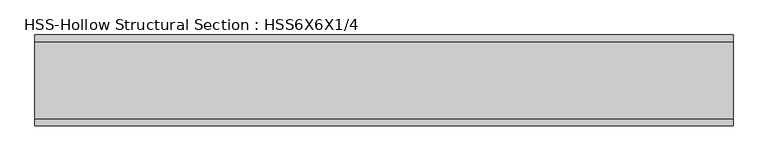
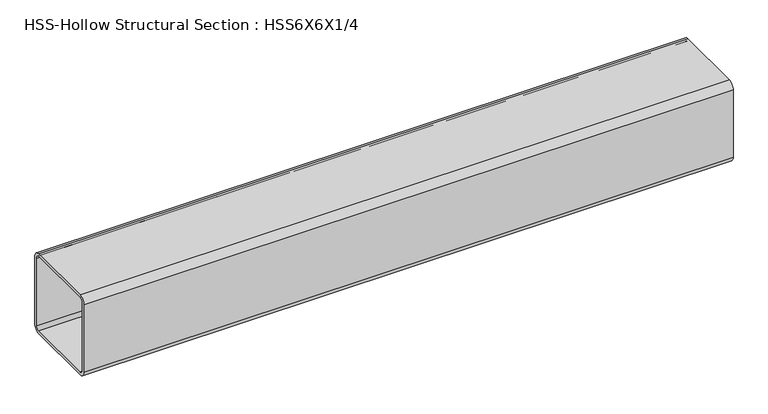
"""IFC4 building model written with IfcOpenShell, lengths in millimetres: beam geometry, HSS-Hollow Structural Section : HSS6X6X1/4."""

from ifc_helpers import new_model, si_unit, point, frame, frame_2d, origin, place, context, project, spatial, polyline, circle_curve, trimmed, segment, composite_curve, outline, extrude, source, transform, mapped, element, save


def hss_hollow_structural_section_hss6x6x1_4_3c38727f(model_context):
    return source(origin(), model_context, "Body", "SweptSolid", [
        extrude(outline(composite_curve([segment(polyline([(76.2, 64.3636), (76.2, -64.3636)]), True, "CONTINUOUS"), segment(trimmed(circle_curve(frame_2d((64.3636, -64.3636)), 11.8364), [point((76.2, -64.3636))], [point((64.3636, -76.2))], False, "CARTESIAN"), True, "CONTINUOUS"), segment(polyline([(64.3636, -76.2), (-64.3636, -76.2)]), True, "CONTINUOUS"), segment(trimmed(circle_curve(frame_2d((-64.3636, -64.3636)), 11.8364), [point((-64.3636, -76.2))], [point((-76.2, -64.3636))], False, "CARTESIAN"), True, "CONTINUOUS"), segment(polyline([(-76.2, -64.3636), (-76.2, 64.3636)]), True, "CONTINUOUS"), segment(trimmed(circle_curve(frame_2d((-64.3636, 64.3636)), 11.8364), [point((-76.2, 64.3636))], [point((-64.3636, 76.2))], False, "CARTESIAN"), True, "CONTINUOUS"), segment(polyline([(-64.3636, 76.2), (64.3636, 76.2)]), True, "CONTINUOUS"), segment(trimmed(circle_curve(frame_2d((64.3636, 64.3636)), 11.8364), [point((64.3636, 76.2))], [point((76.2, 64.3636))], False, "CARTESIAN"), True, "CONTINUOUS")], self_intersect=False), holes=[composite_curve([segment(trimmed(circle_curve(frame_2d((-64.3636, 64.3636)), 5.9182), [point((-64.3636, 70.2818))], [point((-70.2818, 64.3636))], True, "CARTESIAN"), True, "CONTINUOUS"), segment(polyline([(-70.2818, 64.3636), (-70.2818, -64.3636)]), True, "CONTINUOUS"), segment(trimmed(circle_curve(frame_2d((-64.3636, -64.3636)), 5.9182), [point((-70.2818, -64.3636))], [point((-64.3636, -70.2818))], True, "CARTESIAN"), True, "CONTINUOUS"), segment(polyline([(-64.3636, -70.2818), (64.3636, -70.2818)]), True, "CONTINUOUS"), segment(trimmed(circle_curve(frame_2d((64.3636, -64.3636)), 5.9182), [point((64.3636, -70.2818))], [point((70.2818, -64.3636))], True, "CARTESIAN"), True, "CONTINUOUS"), segment(polyline([(70.2818, -64.3636), (70.2818, 64.3636)]), True, "CONTINUOUS"), segment(trimmed(circle_curve(frame_2d((64.3636, 64.3636)), 5.9182), [point((70.2818, 64.3636))], [point((64.3636, 70.2818))], True, "CARTESIAN"), True, "CONTINUOUS"), segment(polyline([(64.3636, 70.2818), (-64.3636, 70.2818)]), True, "CONTINUOUS")], self_intersect=False)]), frame((-637.9810512, 0.0, 0.0), z_axis=(1.0, 0.0, 0.0), x_axis=(0.0, 1.0, 0.0)), (0.0, 0.0, 1.0), 1168.3980486),
    ])


if __name__ == "__main__":
    model = new_model("IFC4")
    model_context = context("Model", 3, world=origin())
    ifc_project = project(units=[si_unit("LENGTHUNIT", "METRE", prefix="MILLI")], contexts=[model_context])
    site = spatial("IfcSite", under=ifc_project)
    building = spatial("IfcBuilding", under=site)
    placement = place(None, origin())
    hss_hollow_structural_section_hss6x6x1_4_shape = hss_hollow_structural_section_hss6x6x1_4_3c38727f(model_context)
    element("IfcBeam", 1, ObjectType="HSS-Hollow Structural Section : HSS6X6X1/4", at=placement, inside=building, context=model_context, shape_type="MappedRepresentation", body=[
        mapped(hss_hollow_structural_section_hss6x6x1_4_shape, transform((0.0, 0.0, 0.0), x_axis=(1.0, 0.0, 0.0), y_axis=(0.0, 1.0, 0.0), z_axis=(0.0, 0.0, 1.0))),
    ])
    save(model, "model.ifc")

# Revit data of these elements
# Type "HSS-Hollow Structural Section : HSS6X6X1/4"
#   Assembly Code = "B10"
#   Shape = "Square"
#   W = 19
#   Ht = 0' - 6"
#   Length [instance default] = 5' - 0"
#   b = 0' - 6"
#   kr = 0' - 0.466"
#   t = 0' - 0.233"
#   A = 0.0363889 SF
#   Structural Material [instance default] = Steel ASTM A500, Grade B, Rectangular and Square
# Element 1 (IfcBeam, "HSS-Hollow Structural Section : HSS6X6X1/4")
#   Materials on its faces: "Steel ASTM A500, Grade B, Rectangular and Square"
# Materials
#   "Steel ASTM A500, Grade B, Rectangular and Square": class "Metal", colour RGB 199 199 199, transparency 0, Description = "Carbon steel", Cost = 0
